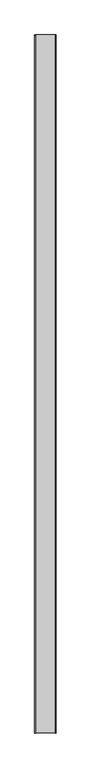
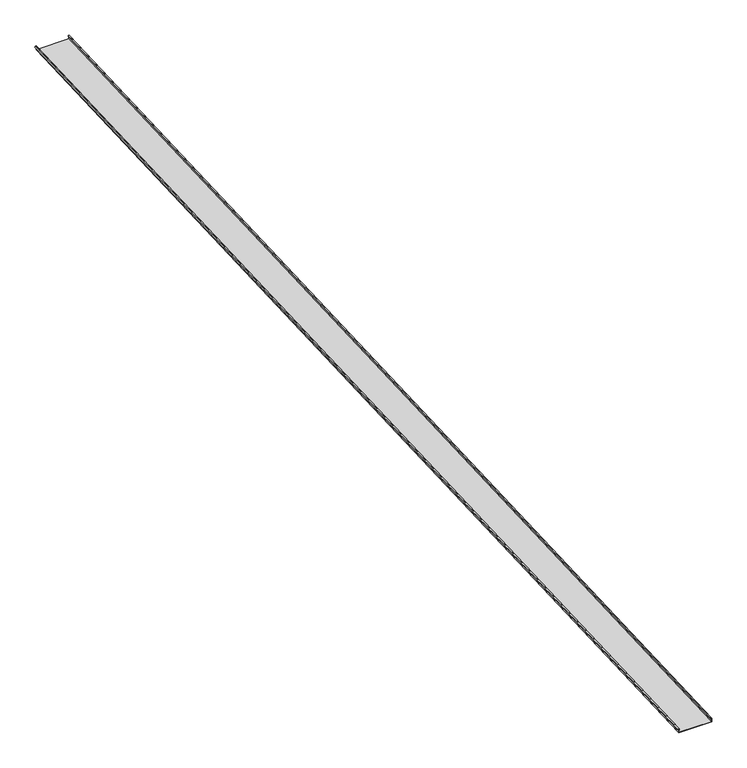
"""IFC4 building model written with IfcOpenShell, lengths in millimetres: proxy geometry, Generic Models 2:Generic Models 2:310765:Generic Models 2:310765 : Generic Models 2:Generic Models 2:310765:14 : Generic Models 2:Generic Models 2:310765:Generic Models 2:310765 : Generic Models 2:Generic Models 2:310765:300385."""

from ifc_helpers import new_model, si_unit, frame, origin, place, context, project, spatial, polyline, outline, extrude, source, transform, mapped, element, save


def generic_models_a39602ba(model_context):
    return source(origin(), model_context, "Body", "SweptSolid", [
        extrude(outline(polyline([(1.5875, 0.0), (1.5875, 50.8), (407.9875, 50.8), (407.9875, 1.5874999), (396.875, 1.5874999), (396.875, 11.1125), (398.4625, 11.1125), (398.4625, 3.175), (406.4, 3.175), (406.4, 49.2125), (3.175, 49.2125), (3.175, -1.5875), (-14.2875, -1.5875), (-14.2875, 9.525), (-12.7, 9.525), (-12.7, 0.0), (1.5875, 0.0)])), frame((592719.1763073, -582045.9363143, 3873.8572241), z_axis=(0.0, 0.9991330730923568, 0.04163054471206784), x_axis=(1.0, 0.0, 0.0)), (0.0, 0.0, 1.0), 13804.8185035),
    ])


if __name__ == "__main__":
    model = new_model("IFC4")
    model_context = context("Model", 3, world=origin())
    ifc_project = project(units=[si_unit("LENGTHUNIT", "METRE", prefix="MILLI")], contexts=[model_context])
    site = spatial("IfcSite", under=ifc_project)
    building = spatial("IfcBuilding", under=site)
    placement = place(None, origin())
    generic_models_shape = generic_models_a39602ba(model_context)
    element("IfcBuildingElementProxy", 1, Name="Generic Models 2:Generic Models 2:310765:Generic Models 2:310765 : Generic Models 2:Generic Models 2:310765:14 : Generic Models 2:Generic Models 2:310765:Generic Models 2:310765 : Generic Models 2:Generic Models 2:310765:300385", ObjectType="Generic Models 2:Generic Models 2:310765:Generic Models 2:310765 : Generic Models 2:Generic Models 2:310765:14 : Generic Models 2:Generic Models 2:310765:Generic Models 2:310765 : Generic Models 2:Generic Models 2:310765:300385", at=placement, inside=building, context=model_context, shape_type="MappedRepresentation", body=[
        mapped(generic_models_shape, transform((0.0, 0.0, 0.0), x_axis=(1.0, 0.0, 0.0), y_axis=(0.0, 1.0, 0.0), z_axis=(0.0, 0.0, 1.0))),
    ])
    save(model, "model.ifc")

# Revit data of these elements
# Type "Generic Models 2:Generic Models 2:310765:Generic Models 2:310765 : Generic Models 2:Generic Models 2:310765:14 : Generic Models 2:Generic Models 2:310765:Generic Models 2:310765 : Generic Models 2:Generic Models 2:310765:300385"
#   NameOverride = "Generic Models 2:Generic Models 2:310765:Generic Models 2:310765 : Generic Models 2:Generic Models 2:310765:300385"
#   ObjectTypeOverride = "Generic Models 2:310765 : Generic Models 2:Generic Models 2:310765"
#   Reference = "Generic Models 2"
#   Tag = "300385"
# Element 1 (IfcBuildingElementProxy, "Generic Models 2:Generic Models 2:310765:Generic Models 2:310765 : Generic Models 2:Generic Models 2:310765:14 : Generic Models 2:Generic Models 2:310765:Generic Models 2:310765 : Generic Models 2:Generic Models 2:310765:300385")
#   Materials on its faces: "STRUCTURAL STANDING SEAM SHEET METAL ROOFING - BATTENLOK - COLOR T.B.D."
# Materials
#   "STRUCTURAL STANDING SEAM SHEET METAL ROOFING - BATTENLOK - COLOR T.B.D.": class "Generic", colour RGB 120 120 120, transparency 0, Cost = 0
